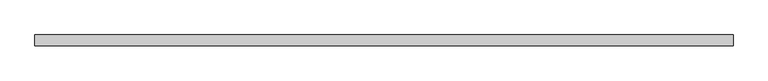
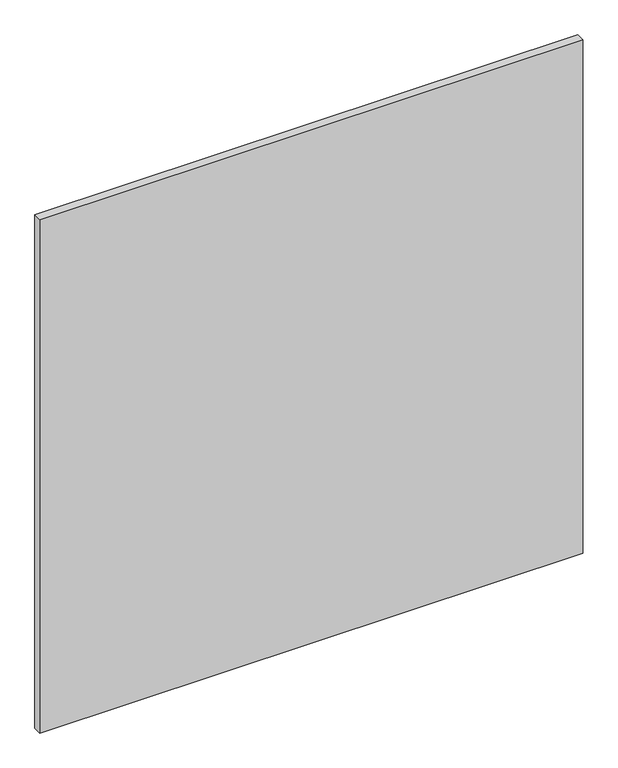
"""IFC4 building model written with IfcOpenShell, lengths in millimetres: proxy geometry, Inner panel:Inner panel:1:Inner panel:1 : Inner panel:Inner panel:300324:300043:Inner panel:1:Inner panel:1 : Inner panel:Inner panel:300324:300043 : Inner panel:Inner panel:1:Inner panel:1 : Inner panel:Inner panel:300324:300043:2 : Inner panel:Inner panel:1:Inner panel:1 : Inner panel:Inner panel:300324:300043:Inner panel:1:Inner panel:1 : Inner panel:Inner panel:300324:300043 : Inner panel:Inner panel:1:Inner panel:1 : Inner panel:Inner panel:300324:300043:300031."""

from ifc_helpers import new_model, si_unit, frame, origin, place, context, project, spatial, polyline, outline, extrude, source, transform, mapped, element, save


def generic_models_3ae2aa65(model_context):
    return source(origin(), model_context, "Body", "SweptSolid", [
        extrude(outline(polyline([(593738.0867239, -578778.4413841), (594957.2867239, -578778.4413841), (594957.2867239, -578797.4913841), (593738.0867239, -578797.4913841), (593738.0867239, -578778.4413841)])), frame((0.0, 0.0, 1270.0), z_axis=(0.0, 0.0, 1.0), x_axis=(1.0, 0.0, 0.0)), (0.0, 0.0, 1.0), 1219.2),
    ])


if __name__ == "__main__":
    model = new_model("IFC4")
    model_context = context("Model", 3, world=origin())
    ifc_project = project(units=[si_unit("LENGTHUNIT", "METRE", prefix="MILLI")], contexts=[model_context])
    site = spatial("IfcSite", under=ifc_project)
    building = spatial("IfcBuilding", under=site)
    placement = place(None, origin())
    generic_models_shape = generic_models_3ae2aa65(model_context)
    element("IfcBuildingElementProxy", 1, Name="Inner panel:Inner panel:1:Inner panel:1 : Inner panel:Inner panel:300324:300043:Inner panel:1:Inner panel:1 : Inner panel:Inner panel:300324:300043 : Inner panel:Inner panel:1:Inner panel:1 : Inner panel:Inner panel:300324:300043:2 : Inner panel:Inner panel:1:Inner panel:1 : Inner panel:Inner panel:300324:300043:Inner panel:1:Inner panel:1 : Inner panel:Inner panel:300324:300043 : Inner panel:Inner panel:1:Inner panel:1 : Inner panel:Inner panel:300324:300043:300031", ObjectType="Inner panel:Inner panel:1:Inner panel:1 : Inner panel:Inner panel:300324:300043:Inner panel:1:Inner panel:1 : Inner panel:Inner panel:300324:300043 : Inner panel:Inner panel:1:Inner panel:1 : Inner panel:Inner panel:300324:300043:2 : Inner panel:Inner panel:1:Inner panel:1 : Inner panel:Inner panel:300324:300043:Inner panel:1:Inner panel:1 : Inner panel:Inner panel:300324:300043 : Inner panel:Inner panel:1:Inner panel:1 : Inner panel:Inner panel:300324:300043:300031", at=placement, inside=building, context=model_context, shape_type="MappedRepresentation", body=[
        mapped(generic_models_shape, transform((0.0, 0.0, 0.0), x_axis=(1.0, 0.0, 0.0), y_axis=(0.0, 1.0, 0.0), z_axis=(0.0, 0.0, 1.0))),
    ])
    save(model, "model.ifc")

# Revit data of these elements
# Type "Inner panel:Inner panel:1:Inner panel:1 : Inner panel:Inner panel:300324:300043:Inner panel:1:Inner panel:1 : Inner panel:Inner panel:300324:300043 : Inner panel:Inner panel:1:Inner panel:1 : Inner panel:Inner panel:300324:300043:2 : Inner panel:Inner panel:1:Inner panel:1 : Inner panel:Inner panel:300324:300043:Inner panel:1:Inner panel:1 : Inner panel:Inner panel:300324:300043 : Inner panel:Inner panel:1:Inner panel:1 : Inner panel:Inner panel:300324:300043:300031"
#   NameOverride = "Inner panel:Inner panel:1:Inner panel:1 : Inner panel:Inner panel:300324:300043:Inner panel:1:Inner panel:1 : Inner panel:Inner panel:300324:300043 : Inner panel:Inner panel:1:Inner panel:1 : Inner panel:Inner panel:300324:300043:300031"
#   ObjectTypeOverride = "Inner panel:1:Inner panel:1 : Inner panel:Inner panel:300324:300043 : Inner panel:Inner panel:1:Inner panel:1 : Inner panel:Inner panel:300324:300043"
#   Reference = "Inner panel"
#   Tag = "300031"
# Element 1 (IfcBuildingElementProxy, "Inner panel:Inner panel:1:Inner panel:1 : Inner panel:Inner panel:300324:300043:Inner panel:1:Inner panel:1 : Inner panel:Inner panel:300324:300043 : Inner panel:Inner panel:1:Inner panel:1 : Inner panel:Inner panel:300324:300043:2 : Inner panel:Inner panel:1:Inner panel:1 : Inner panel:Inner panel:300324:300043:Inner panel:1:Inner panel:1 : Inner panel:Inner panel:300324:300043 : Inner panel:Inner panel:1:Inner panel:1 : Inner panel:Inner panel:300324:300043:300031")
#   Materials on its faces: "¾” (CLASS A) FIRE RETARDANT PLYWOOD ...OR… IF 1/4\" GYP. BD UNDER PLYWOOD, FLAME SPREAD TO BE CLASS C -  (FINISH: GRADE B - PREFINISHED STAINED/SEALED) - 1/4\" GAP BTWN PANELS (FASTENERS T.B.D.)"
# Materials
#   "¾” (CLASS A) FIRE RETARDANT PLYWOOD ...OR… IF 1/4\" GYP. BD UNDER PLYWOOD, FLAME SPREAD TO BE CLASS C -  (FINISH: GRADE B - PREFINISHED STAINED/SEALED) - 1/4\" GAP BTWN PANELS (FASTENERS T.B.D.)": class "Wood", colour RGB 149 120 74, transparency 0, Description = "Plywood, sheathing grade", Cost = 0
